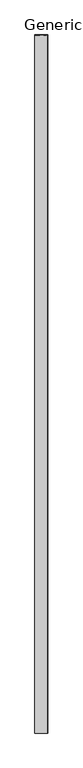
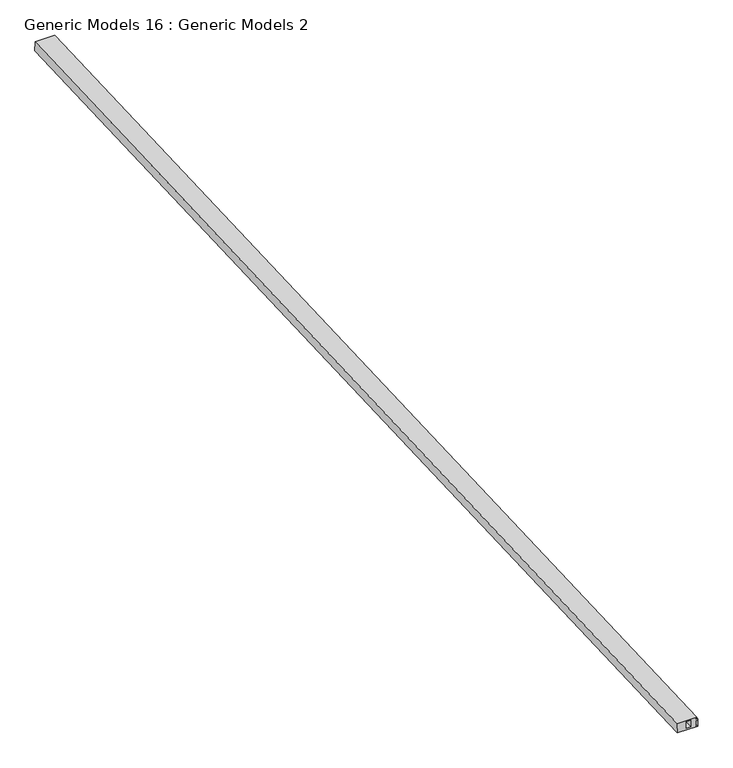
"""IFC4 building model written with IfcOpenShell, lengths in millimetres: proxy geometry, Generic Models 16 : Generic Models 2."""

from ifc_helpers import new_model, si_unit, frame, origin, place, context, project, spatial, polyline, outline, extrude, source, transform, mapped, element, save


def generic_models_16_generic_models_2_80b77924(model_context):
    return source(origin(), model_context, "Body", "SweptSolid", [
        extrude(outline(polyline([(-85.8789767, 0.0), (-9.6789767, 0.0), (-9.6789767, 20.1179581), (-56.5123579, 20.1179581), (-56.5123579, 51.8704763), (529.4252661, 51.8704763), (529.4252661, -243.3629067), (-85.8789767, -243.3629067), (-85.8789767, 0.0)]), holes=[polyline([(122.8066349, 17.3502922), (122.8066349, -187.7883585), (263.9183313, -187.7883585), (263.9183313, 17.3502922), (122.8066349, 17.3502922)]), polyline([(-82.7244048, -240.2755045), (-36.8865501, -240.2755045), (-36.8865501, -50.9035333), (-82.7244048, -50.9035333), (-82.7244048, -240.2755045)])]), frame((667461.4327472, -569964.3689327, 8683.9005509), z_axis=(0.0, 0.9991330730923521, 0.041630544712176844), x_axis=(-1.0, 0.0, 0.0)), (0.0, 0.0, 1.0), 33406.7702703),
    ])


if __name__ == "__main__":
    model = new_model("IFC4")
    model_context = context("Model", 3, world=origin())
    ifc_project = project(units=[si_unit("LENGTHUNIT", "METRE", prefix="MILLI")], contexts=[model_context])
    site = spatial("IfcSite", under=ifc_project)
    building = spatial("IfcBuilding", under=site)
    placement = place(None, origin())
    generic_models_16_generic_models_2_shape = generic_models_16_generic_models_2_80b77924(model_context)
    element("IfcBuildingElementProxy", 1, Name="Generic Models 16 : Generic Models 2", ObjectType="Generic Models 16 : Generic Models 2", at=placement, inside=building, context=model_context, shape_type="MappedRepresentation", body=[
        mapped(generic_models_16_generic_models_2_shape, transform((0.0, 0.0, 0.0), x_axis=(1.0, 0.0, 0.0), y_axis=(0.0, 1.0, 0.0), z_axis=(0.0, 0.0, 1.0))),
    ])
    save(model, "model.ifc")

# Revit data of these elements
# Element 1 (IfcBuildingElementProxy, "Generic Models 16 : Generic Models 2")
#   Materials on its faces: "CLASS A FIBERGLASS INSULATION WITH DURABLE VAPOR BARRIER (WHITE) LINE"
# Materials
#   "CLASS A FIBERGLASS INSULATION WITH DURABLE VAPOR BARRIER (WHITE) LINE": class "Unassigned", colour RGB 187 139 199, transparency 0, Cost = 0
